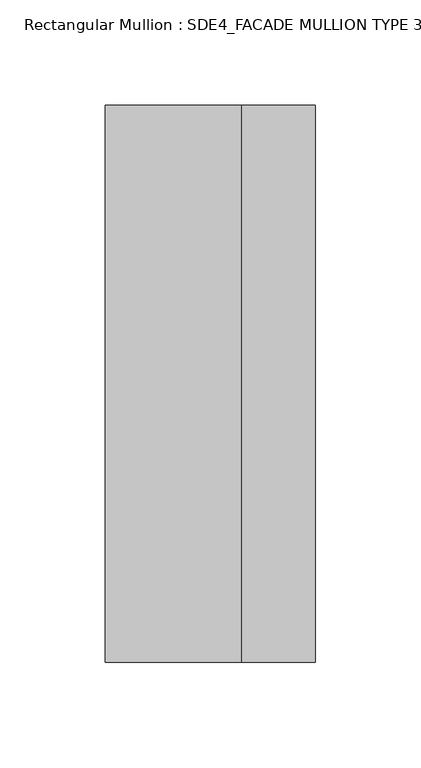
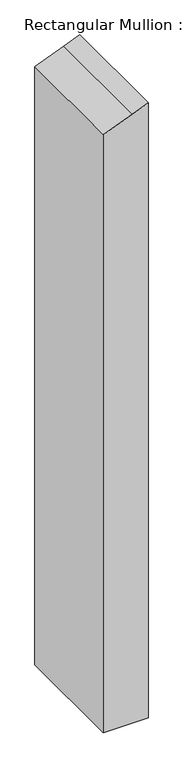
"""IFC4 building model written with IfcOpenShell, lengths in millimetres: member geometry, Rectangular Mullion : SDE4_FACADE MULLION TYPE 3."""

from ifc_helpers import new_model, si_unit, frame, origin, place, context, project, spatial, polyline, outline, extrude, source, transform, mapped, element, save


def rectangular_mullion_sde4_facade_mullion_type_3_06cd8fde(model_context):
    return source(origin(), model_context, "Body", "SweptSolid", [
        extrude(outline(polyline([(-23.0813185, 50.0), (-37.1390676, 14.8556271), (-63.0813185, -50.0), (-1477.974544, -50.0), (-1477.974544, 50.0), (-23.0813185, 50.0)])), frame((0.0, -132.5, 0.0), z_axis=(0.0, 1.0, 0.0), x_axis=(0.0, 0.0, 1.0)), (0.0, 0.0, 1.0), 265.0),
    ])


if __name__ == "__main__":
    model = new_model("IFC4")
    model_context = context("Model", 3, world=origin())
    ifc_project = project(units=[si_unit("LENGTHUNIT", "METRE", prefix="MILLI")], contexts=[model_context])
    site = spatial("IfcSite", under=ifc_project)
    building = spatial("IfcBuilding", under=site)
    placement = place(None, origin())
    rectangular_mullion_sde4_facade_mullion_type_3_shape = rectangular_mullion_sde4_facade_mullion_type_3_06cd8fde(model_context)
    element("IfcMember", 1, ObjectType="Rectangular Mullion : SDE4_FACADE MULLION TYPE 3", at=placement, inside=building, context=model_context, shape_type="MappedRepresentation", body=[
        mapped(rectangular_mullion_sde4_facade_mullion_type_3_shape, transform((0.0, 0.0, 0.0), x_axis=(1.0, 0.0, 0.0), y_axis=(0.0, 1.0, 0.0), z_axis=(0.0, 0.0, 1.0))),
    ])
    save(model, "model.ifc")

# Revit data of these elements
# Type "Rectangular Mullion : SDE4_FACADE MULLION TYPE 3"
#   built-in parameter 1007322 = 0.869423 (stored number, unit not read)
#   built-in parameter 1007321 = 0.164042 (stored number, unit not read)
#   built-in parameter 1007320 = 0.164042 (stored number, unit not read)
